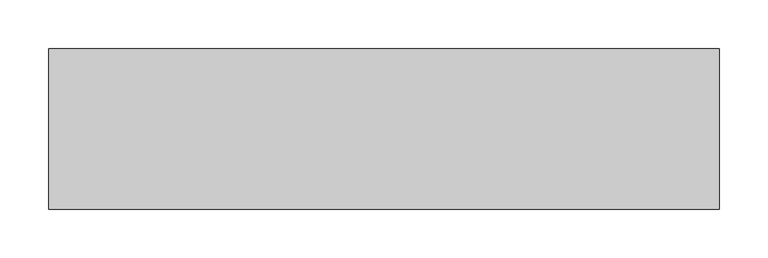
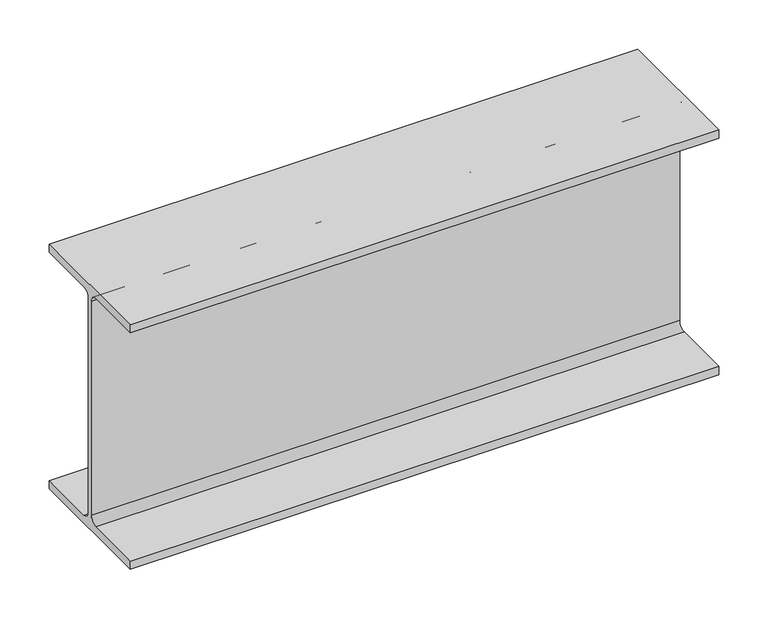
"""IFC4 building model written with IfcOpenShell, lengths in millimetres: beam geometry, Old_Steel Beam_H-KSD3502 : H_SB_ASB_H-300×150x6.5x9."""

from ifc_helpers import new_model, si_unit, point, frame, frame_2d, origin, place, context, project, spatial, polyline, circle_curve, trimmed, segment, composite_curve, outline, extrude, source, transform, mapped, element, save


def beam_9dc301ca(model_context):
    return source(origin(), model_context, "Body", "SweptSolid", [
        extrude(outline(composite_curve([segment(polyline([(82.5, -141.5), (82.5, -151.7), (-82.5, -151.7), (-82.5, -141.5), (-11.9, -141.5)]), True, "CONTINUOUS"), segment(trimmed(circle_curve(frame_2d((-11.9, -132.6)), 8.9), [point((-11.9, -141.5))], [point((-3.0, -132.6))], True, "CARTESIAN"), True, "CONTINUOUS"), segment(polyline([(-3.0, -132.6), (-3.0, 132.6)]), True, "CONTINUOUS"), segment(trimmed(circle_curve(frame_2d((-11.9, 132.6)), 8.9), [point((-3.0, 132.6))], [point((-11.9, 141.5))], True, "CARTESIAN"), True, "CONTINUOUS"), segment(polyline([(-11.9, 141.5), (-82.5, 141.5), (-82.5, 151.7), (82.5, 151.7), (82.5, 141.5), (11.9, 141.5)]), True, "CONTINUOUS"), segment(trimmed(circle_curve(frame_2d((11.9, 132.6)), 8.9), [point((11.9, 141.5))], [point((3.0, 132.6))], True, "CARTESIAN"), True, "CONTINUOUS"), segment(polyline([(3.0, 132.6), (3.0, -132.6)]), True, "CONTINUOUS"), segment(trimmed(circle_curve(frame_2d((11.9, -132.6)), 8.9), [point((3.0, -132.6))], [point((11.9, -141.5))], True, "CARTESIAN"), True, "CONTINUOUS"), segment(polyline([(11.9, -141.5), (82.5, -141.5)]), True, "CONTINUOUS")], self_intersect=False)), frame((-344.9999994, 0.0, 0.0), z_axis=(1.0, 0.0, 0.0), x_axis=(0.0, 1.0, 0.0)), (0.0, 0.0, 1.0), 689.9999994),
    ])


if __name__ == "__main__":
    model = new_model("IFC4")
    model_context = context("Model", 3, world=origin())
    ifc_project = project(units=[si_unit("LENGTHUNIT", "METRE", prefix="MILLI")], contexts=[model_context])
    site = spatial("IfcSite", under=ifc_project)
    building = spatial("IfcBuilding", under=site)
    placement = place(None, origin())
    beam_shape = beam_9dc301ca(model_context)
    element("IfcBeam", 1, ObjectType="Old_Steel Beam_H-KSD3502 : H_SB_ASB_H-300×150x6.5x9", at=placement, inside=building, context=model_context, shape_type="MappedRepresentation", body=[
        mapped(beam_shape, transform((0.0, 0.0, 0.0), x_axis=(1.0, 0.0, 0.0), y_axis=(0.0, 1.0, 0.0), z_axis=(0.0, 0.0, 1.0))),
    ])
    save(model, "model.ifc")

# Revit data of these elements
# Type "Old_Steel Beam_H-KSD3502 : H_SB_ASB_H-300×150x6.5x9"
#   Width = 15.0 cm
#   Web Thickness = 0.65 cm
#   Web Fillet = 1.3 cm
#   Warping Constant = 107174.0 cm⁶
#   Torsional Moment of Inertia = 9.9539 cm⁴
#   Torsional Modulus = 1.0 cm³
#   Section Area = 46.78 cm²
#   Plastic Modulus weak axis = 105.0 cm³
#   Plastic Modulus strong axis = 542.0 cm³
#   Perimeter = 1.17 m²/m
#   Nominal Weight = 36.70 kgf/m
#   Moment of Inertia weak axis = 508.00 cm⁴
#   Moment of Inertia strong axis = 7210.00 cm⁴
#   Height = 30.0 cm
#   Flange Thickness = 0.9 cm
#   Elastic Modulus weak axis = 67.7 cm³
#   Elastic Modulus strong axis = 481.0 cm³
#   Centroid Vertical = 15.0 cm
#   Centroid Horizontal = 7.5 cm
#   Length [instance default] = 1.5240 m
#   Structural Material [instance default] = Steel, 45-345
#   Assembly Code = ""
# Element 1 (IfcBeam, "Old_Steel Beam_H-KSD3502 : H_SB_ASB_H-300×150x6.5x9")
#   Structural Material = none
# Materials
#   "Steel, 45-345": class "Metal", colour RGB 189 187 185, transparency 0, Description = "Steel 345 MPa", Cost = 0
